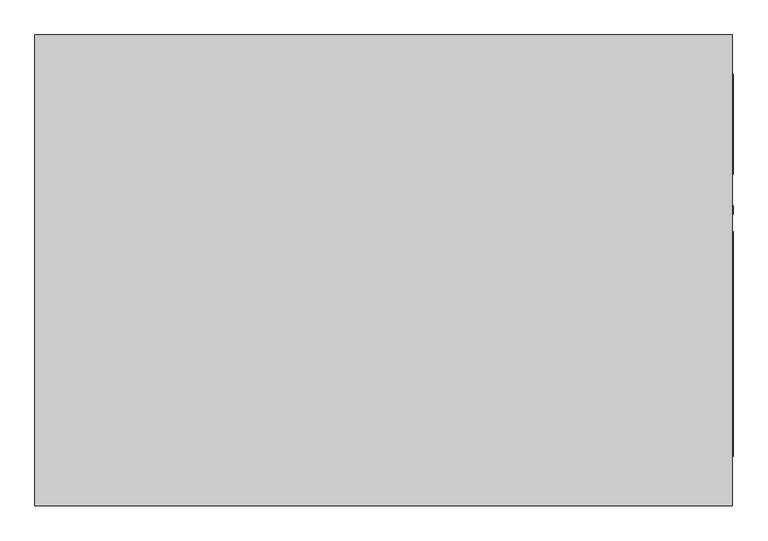
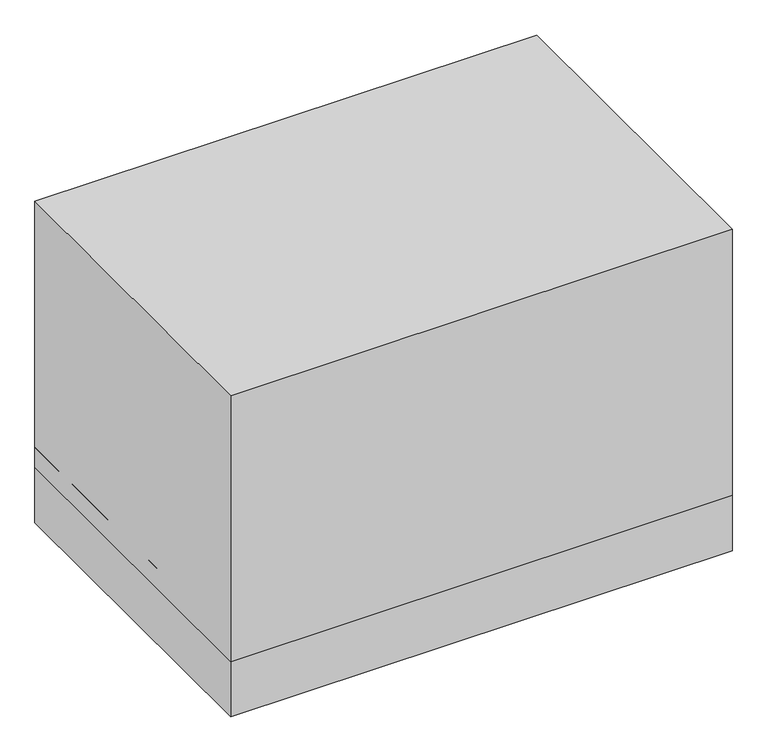
"""IFC4 building model written with IfcOpenShell, lengths in millimetres: proxy geometry, Carrier_48TC_Standard_Efficiency_Gas_Heat_Electric_Cooling_Packaged_Rooftop_Unit_3_to_15_nominal_tons : 10 ton 48TC**12."""

from ifc_helpers import new_model, si_unit, point, frame, frame_2d, origin, origin_with_axes, place, context, project, spatial, polyline, circle_curve, trimmed, segment, composite_curve, outline, extrude, source, transform, mapped, element, save
from ifc_brep_helpers import plane_surface, revolved_surface, advanced_brep


def mechanical_equipment_e741c091(model_context):
    return source(origin(), model_context, "Body", "SolidModel", [
        extrude(outline(composite_curve([segment(trimmed(circle_curve(frame_2d((193.675, 438.15)), 13.2953125), [point((180.3796875, 438.15))], [point((206.9703125, 438.15))], False, "CARTESIAN"), True, "CONTINUOUS"), segment(trimmed(circle_curve(frame_2d((193.675, 438.15)), 13.2953125), [point((206.9703125, 438.15))], [point((180.3796875, 438.15))], False, "CARTESIAN"), True, "CONTINUOUS")], self_intersect=False)), frame((1119.1875, 0.0, 0.0), z_axis=(1.0, 0.0, 0.0), x_axis=(0.0, 1.0, 0.0)), (0.0, 0.0, 1.0), 3.175),
        advanced_brep(
        [(1119.1875, 755.65, 1514.475), (-1119.1875, 755.65, 1514.475), (-1119.1875, -755.65, 1514.475), (1119.1875, -755.65, 1514.475), (1119.1875, 755.65, 260.35), (1119.1875, -755.65, 260.35), (-1119.1875, -755.65, 260.35), (-1119.1875, 755.65, 260.35), (1036.6375, -596.9, 260.35), (1036.6375, 133.35, 260.35), (681.0375, 133.35, 260.35), (681.0375, -596.9, 260.35), (1036.6375, 590.55, 260.35), (112.7125, 590.55, 260.35), (112.7125, 269.875, 260.35), (1036.6375, 269.875, 260.35), (176.8078125, -107.95, 260.35), (150.2171875, -107.95, 260.35), (-355.6, -476.25, 260.35), (-377.825, -476.25, 260.35), (-344.4875, -349.25, 260.35), (-388.9375, -349.25, 260.35), (-344.4875, -298.45, 260.35), (-388.9375, -298.45, 260.35), (1036.6375, -596.9, 381.0), (681.0375, -596.9, 381.0), (681.0375, 133.35, 381.0), (1036.6375, 133.35, 381.0), (1036.6375, 590.55, 381.0), (1036.6375, 269.875, 381.0), (112.7125, 269.875, 381.0), (112.7125, 590.55, 381.0), (176.8078125, -107.95, 406.4), (150.2171875, -107.95, 406.4), (-355.6, -476.25, 406.4), (-377.825, -476.25, 406.4), (-344.4875, -349.25, 406.4), (-388.9375, -349.25, 406.4), (-344.4875, -298.45, 406.4), (-388.9375, -298.45, 406.4)],
        [
            (0, 1),
            (1, 2),
            (2, 3),
            (3, 0),
            (4, 5),
            (5, 6),
            (6, 7),
            (7, 4),
            (8, 9),
            (9, 10),
            (10, 11),
            (11, 8),
            (12, 13),
            (13, 14),
            (14, 15),
            (15, 12),
            (16, 17, circle_curve(frame((163.5125, -107.95, 260.35), z_axis=(0.0, 0.0, 1.0), x_axis=(-1.0, 0.0, 0.0)), 13.2953125)),
            (17, 16, circle_curve(frame((163.5125, -107.95, 260.35), z_axis=(0.0, 0.0, 1.0), x_axis=(-1.0, 0.0, 0.0)), 13.2953125)),
            (18, 19, circle_curve(frame((-366.7125, -476.25, 260.35), z_axis=(0.0, 0.0, 1.0), x_axis=(-1.0, 0.0, 0.0)), 11.1125)),
            (19, 18, circle_curve(frame((-366.7125, -476.25, 260.35), z_axis=(0.0, 0.0, 1.0), x_axis=(-1.0, 0.0, 0.0)), 11.1125)),
            (20, 21, circle_curve(frame((-366.7125, -349.25, 260.35), z_axis=(0.0, 0.0, 1.0), x_axis=(-1.0, 0.0, 0.0)), 22.225)),
            (21, 20, circle_curve(frame((-366.7125, -349.25, 260.35), z_axis=(0.0, 0.0, 1.0), x_axis=(-1.0, 0.0, 0.0)), 22.225)),
            (22, 23, circle_curve(frame((-366.7125, -298.45, 260.35), z_axis=(0.0, 0.0, 1.0), x_axis=(-1.0, 0.0, 0.0)), 22.225)),
            (23, 22, circle_curve(frame((-366.7125, -298.45, 260.35), z_axis=(0.0, 0.0, 1.0), x_axis=(-1.0, 0.0, 0.0)), 22.225)),
            (0, 4),
            (7, 1),
            (6, 2),
            (5, 3),
            (24, 25),
            (25, 26),
            (26, 27),
            (27, 24),
            (27, 9),
            (8, 24),
            (26, 10),
            (25, 11),
            (28, 29),
            (29, 30),
            (30, 31),
            (31, 28),
            (31, 13),
            (12, 28),
            (30, 14),
            (29, 15),
            (32, 33, circle_curve(frame((163.5125, -107.95, 406.4), z_axis=(0.0, 0.0, -1.0), x_axis=(-1.0, 0.0, 0.0)), 13.2953125)),
            (33, 32, circle_curve(frame((163.5125, -107.95, 406.4), z_axis=(0.0, 0.0, -1.0), x_axis=(-1.0, 0.0, 0.0)), 13.2953125)),
            (33, 17),
            (16, 32),
            (34, 35, circle_curve(frame((-366.7125, -476.25, 406.4), z_axis=(0.0, 0.0, -1.0), x_axis=(-1.0, 0.0, 0.0)), 11.1125)),
            (35, 34, circle_curve(frame((-366.7125, -476.25, 406.4), z_axis=(0.0, 0.0, -1.0), x_axis=(-1.0, 0.0, 0.0)), 11.1125)),
            (35, 19),
            (18, 34),
            (36, 37, circle_curve(frame((-366.7125, -349.25, 406.4), z_axis=(0.0, 0.0, -1.0), x_axis=(-1.0, 0.0, 0.0)), 22.225)),
            (37, 36, circle_curve(frame((-366.7125, -349.25, 406.4), z_axis=(0.0, 0.0, -1.0), x_axis=(-1.0, 0.0, 0.0)), 22.225)),
            (37, 21),
            (20, 36),
            (38, 39, circle_curve(frame((-366.7125, -298.45, 406.4), z_axis=(0.0, 0.0, -1.0), x_axis=(-1.0, 0.0, 0.0)), 22.225)),
            (39, 38, circle_curve(frame((-366.7125, -298.45, 406.4), z_axis=(0.0, 0.0, -1.0), x_axis=(-1.0, 0.0, 0.0)), 22.225)),
            (39, 23),
            (22, 38),
        ],
        [
            plane_surface(frame((-1119.1875, 755.65, 1514.475), z_axis=(0.0, 0.0, 1.0), x_axis=(-1.0, 0.0, 0.0))),
            plane_surface(frame((-1119.1875, 755.65, 260.35), z_axis=(0.0, 0.0, -1.0), x_axis=(1.0, 0.0, 0.0))),
            plane_surface(frame((1119.1875, 755.65, 1514.475), z_axis=(0.0, 1.0, 0.0), x_axis=(0.0, 0.0, -1.0))),
            plane_surface(frame((-1119.1875, 755.65, 1514.475), z_axis=(-1.0, 0.0, 0.0), x_axis=(0.0, 0.0, -1.0))),
            plane_surface(frame((-1119.1875, -755.65, 1514.475), z_axis=(0.0, -1.0, 0.0), x_axis=(0.0, 0.0, -1.0))),
            plane_surface(frame((1119.1875, -755.65, 1514.475), z_axis=(1.0, 0.0, 0.0), x_axis=(0.0, 0.0, -1.0))),
            plane_surface(frame((1036.6375, -596.9, 381.0), z_axis=(0.0, 0.0, -1.0), x_axis=(0.0, 1.0, 0.0))),
            plane_surface(frame((1036.6375, -596.9, 381.0), z_axis=(-1.0, 0.0, 0.0), x_axis=(0.0, 0.0, -1.0))),
            plane_surface(frame((1036.6375, 133.35, 381.0), z_axis=(0.0, -1.0, 0.0), x_axis=(0.0, 0.0, -1.0))),
            plane_surface(frame((681.0375, 133.35, 381.0), z_axis=(1.0, 0.0, 0.0), x_axis=(0.0, 0.0, -1.0))),
            plane_surface(frame((681.0375, -596.9, 381.0), z_axis=(0.0, 1.0, 0.0), x_axis=(0.0, 0.0, -1.0))),
            plane_surface(frame((112.7125, 590.55, 381.0), z_axis=(0.0, 0.0, -1.0), x_axis=(-1.0, 0.0, 0.0))),
            plane_surface(frame((1036.6375, 590.55, 381.0), z_axis=(0.0, -1.0, 0.0), x_axis=(0.0, 0.0, -1.0))),
            plane_surface(frame((112.7125, 590.55, 381.0), z_axis=(1.0, 0.0, 0.0), x_axis=(0.0, 0.0, -1.0))),
            plane_surface(frame((112.7125, 269.875, 381.0), z_axis=(0.0, 1.0, 0.0), x_axis=(0.0, 0.0, -1.0))),
            plane_surface(frame((1036.6375, 269.875, 381.0), z_axis=(-1.0, 0.0, 0.0), x_axis=(0.0, 0.0, -1.0))),
            plane_surface(frame((150.2171875, -107.95, 406.4), z_axis=(0.0, 0.0, -1.0), x_axis=(0.0, -1.0, 0.0))),
            revolved_surface(polyline([(150.2171875, -107.95, 406.4), (150.2171875, -107.95, 260.35)]), (163.5125, -107.95, 0.0), (0.0, 0.0, 1.0)),
            plane_surface(frame((-377.825, -476.25, 406.4), z_axis=(0.0, 0.0, -1.0), x_axis=(0.0, -1.0, 0.0))),
            revolved_surface(polyline([(-377.825, -476.25, 406.4), (-377.825, -476.25, 260.35)]), (-366.7125, -476.25, 0.0), (0.0, 0.0, 1.0)),
            plane_surface(frame((-388.9375, -349.25, 406.4), z_axis=(0.0, 0.0, -1.0), x_axis=(0.0, -1.0, 0.0))),
            revolved_surface(polyline([(-388.9375, -349.25, 406.4), (-388.9375, -349.25, 260.35)]), (-366.7125, -349.25, 0.0), (0.0, 0.0, 1.0)),
            plane_surface(frame((-388.9375, -298.45, 406.4), z_axis=(0.0, 0.0, -1.0), x_axis=(0.0, -1.0, 0.0))),
            revolved_surface(polyline([(-388.9375, -298.45, 406.4), (-388.9375, -298.45, 260.35)]), (-366.7125, -298.45, 0.0), (0.0, 0.0, 1.0)),
        ],
        [
            (0, [[1, 2, 3, 4]]),
            (1, [[5, 6, 7, 8], [9, 10, 11, 12], [13, 14, 15, 16], [17, 18], [19, 20], [21, 22], [23, 24]]),
            (2, [[-1, 25, -8, 26]]),
            (3, [[-2, -26, -7, 27]]),
            (4, [[-3, -27, -6, 28]]),
            (5, [[-4, -28, -5, -25]]),
            (6, [[29, 30, 31, 32]]),
            (7, [[-32, 33, -9, 34]]),
            (8, [[-31, 35, -10, -33]]),
            (9, [[-30, 36, -11, -35]]),
            (10, [[-29, -34, -12, -36]]),
            (11, [[37, 38, 39, 40]]),
            (12, [[-40, 41, -13, 42]]),
            (13, [[-39, 43, -14, -41]]),
            (14, [[-38, 44, -15, -43]]),
            (15, [[-37, -42, -16, -44]]),
            (16, [[45, 46]]),
            (17, [[-46, 47, -17, 48]]),
            (17, [[-45, -48, -18, -47]]),
            (18, [[49, 50]]),
            (19, [[-50, 51, -19, 52]]),
            (19, [[-49, -52, -20, -51]]),
            (20, [[53, 54]]),
            (21, [[-54, 55, -21, 56]]),
            (21, [[-53, -56, -22, -55]]),
            (22, [[57, 58]]),
            (23, [[-58, 59, -23, 60]]),
            (23, [[-57, -60, -24, -59]]),
        ],
    ),
        extrude(outline(polyline([(1119.1875, 755.65), (1119.1875, -755.65), (-1119.1875, -755.65), (-1119.1875, 755.65), (1119.1875, 755.65)]), holes=[polyline([(1036.6375, 590.55), (112.7125, 590.55), (112.7125, 269.875), (1036.6375, 269.875), (1036.6375, 590.55)]), polyline([(1036.6375, -596.9), (1036.6375, 133.35), (681.0375, 133.35), (681.0375, -596.9), (1036.6375, -596.9)]), composite_curve([segment(trimmed(circle_curve(frame_2d((163.5125, -107.95)), 13.2953125), [point((176.8078125, -107.95))], [point((150.2171875, -107.95))], True, "CARTESIAN"), True, "CONTINUOUS"), segment(trimmed(circle_curve(frame_2d((163.5125, -107.95)), 13.2953125), [point((150.2171875, -107.95))], [point((176.8078125, -107.95))], True, "CARTESIAN"), True, "CONTINUOUS")], self_intersect=False), composite_curve([segment(trimmed(circle_curve(frame_2d((-366.7125, -476.25)), 11.1125), [point((-355.6, -476.25))], [point((-377.825, -476.25))], True, "CARTESIAN"), True, "CONTINUOUS"), segment(trimmed(circle_curve(frame_2d((-366.7125, -476.25)), 11.1125), [point((-377.825, -476.25))], [point((-355.6, -476.25))], True, "CARTESIAN"), True, "CONTINUOUS")], self_intersect=False), composite_curve([segment(trimmed(circle_curve(frame_2d((-366.7125, -349.25)), 22.225), [point((-344.4875, -349.25))], [point((-388.9375, -349.25))], True, "CARTESIAN"), True, "CONTINUOUS"), segment(trimmed(circle_curve(frame_2d((-366.7125, -349.25)), 22.225), [point((-388.9375, -349.25))], [point((-344.4875, -349.25))], True, "CARTESIAN"), True, "CONTINUOUS")], self_intersect=False), composite_curve([segment(trimmed(circle_curve(frame_2d((-366.7125, -298.45)), 22.225), [point((-344.4875, -298.45))], [point((-388.9375, -298.45))], True, "CARTESIAN"), True, "CONTINUOUS"), segment(trimmed(circle_curve(frame_2d((-366.7125, -298.45)), 22.225), [point((-388.9375, -298.45))], [point((-344.4875, -298.45))], True, "CARTESIAN"), True, "CONTINUOUS")], self_intersect=False)]), origin_with_axes(), (0.0, 0.0, 1.0), 355.6),
        extrude(outline(polyline([(1122.3625, 628.65), (1122.3625, 307.975), (1119.1875, 307.975), (1119.1875, 628.65), (1122.3625, 628.65)])), frame((0.0, 0.0, 406.4), z_axis=(0.0, 0.0, 1.0), x_axis=(1.0, 0.0, 0.0)), (0.0, 0.0, 1.0), 923.925),
        extrude(outline(polyline([(1122.3625, 123.825), (1122.3625, -596.9), (1119.1875, -596.9), (1119.1875, 123.825), (1122.3625, 123.825)])), frame((0.0, 0.0, 406.4), z_axis=(0.0, 0.0, 1.0), x_axis=(1.0, 0.0, 0.0)), (0.0, 0.0, 1.0), 352.425),
    ])


if __name__ == "__main__":
    model = new_model("IFC4")
    model_context = context("Model", 3, world=origin())
    ifc_project = project(units=[si_unit("LENGTHUNIT", "METRE", prefix="MILLI")], contexts=[model_context])
    site = spatial("IfcSite", under=ifc_project)
    building = spatial("IfcBuilding", under=site)
    placement = place(None, origin())
    mechanical_equipment_shape = mechanical_equipment_e741c091(model_context)
    element("IfcBuildingElementProxy", 1, Name="Carrier_48TC_Standard_Efficiency_Gas_Heat_Electric_Cooling_Packaged_Rooftop_Unit_3_to_15_nominal_tons : 10 ton 48TC**12", ObjectType="Carrier_48TC_Standard_Efficiency_Gas_Heat_Electric_Cooling_Packaged_Rooftop_Unit_3_to_15_nominal_tons : 10 ton 48TC**12", at=placement, inside=building, context=model_context, shape_type="MappedRepresentation", body=[
        mapped(mechanical_equipment_shape, transform((0.0, 0.0, 0.0), x_axis=(1.0, 0.0, 0.0), y_axis=(0.0, 1.0, 0.0), z_axis=(0.0, 0.0, 1.0))),
    ])
    save(model, "model.ifc")

# Revit data of these elements
# Type "Carrier_48TC_Standard_Efficiency_Gas_Heat_Electric_Cooling_Packaged_Rooftop_Unit_3_to_15_nominal_tons : 10 ton 48TC**12"
#   URL = "www.Carrier.com"
#   Model = "48TC"
#   Manufacturer = "Carrier"
#   Disclaimer = "Manufacturer reserves the right to change, at any time, specifications and designs without notice and without obligation.  Please verify critical parameters with local Carrier commercial sales office."
#   knockout thickness = 0' - 0 1/16"
#   Voltage = 0 V
#   Version = 1
#   TTBY3 = 0' - 11"
#   TTBY2 = 1' - 4"
#   TTBY1 = 1' - 6"
#   TTBX = 2' - 5 5/8"
#   TTBPowerR = 0' - 0 7/8"
#   TTBGasR = 0' - 0 7/8"
#   SSSZ = 0' - 5 3/4"
#   SSSY = 0' - 6 1/4"
#   SSSW = 2' - 4 3/8"
#   SSSH = 1' - 1 7/8"
#   SSRZ = 0' - 5 3/4"
#   SSRY = 0' - 5"
#   SSRW = 1' - 0 5/8"
#   SSRH = 3' - 0 3/8"
#   SEER = 0
#   Right clearance = 3' - 0"
#   PWRZ = 2' - 3 7/8"
#   PWRY = 0' - 4 5/8"
#   PWRR = 0' - 1 1/4"
#   ODF2X = 1' - 0"
#   ODF1Y = 0' - 11"
#   ODF1X = 2' - 1"
#   ODF1R = 0' - 10"
#   MOCP = 0 A
#   MCA = 0 A
#   Left clearance = 4' - 0"
#   IEER = 11.8
#   Front clearance = 4' - 0"
#   Fan Z = 4' - 11 5/8"
#   Width = 4' - 11 1/2"
#   Length = 7' - 4 1/8"
#   Height = 4' - 1 3/8"
#   EER = 11.1
#   DSSY = 0' - 6 1/4"
#   DSSX = 0' - 3 1/4"
#   DSSW = 1' - 2"
#   DSSH = 2' - 4 3/4"
#   DSRY = 0' - 6 1/2"
#   DSRX = 0' - 3 1/4"
#   DSRW = 3' - 0 3/8"
#   DSRH = 1' - 0 5/8"
#   DRNZ = 0' - 7"
#   DRNY = 3' - 1 3/8"
#   DRNR = 0' - 0 67/128"
#   Curb Z = 1' - 2"
#   CFM (nominal) = 0 CFM
#   Back clearance = 3' - 0"
#   Alt Condensate Drain = 0' - 0 67/128"
#   AccypwrR = 0' - 0 7/16"
#   ACY = 2' - 1 1/2"
#   ACX = 3' - 1 5/8"
#   Gas [instance default] = yes
#   Fan 2 on = yes
#   Curb_1SLAB_2ROOFCURB_3SNOWCURB = 2
#   Fan 3 on = no
#   Unit material = RTU
#   Curb material = Curb paint
# Element 1 (IfcBuildingElementProxy, "Carrier_48TC_Standard_Efficiency_Gas_Heat_Electric_Cooling_Packaged_Rooftop_Unit_3_to_15_nominal_tons : 10 ton 48TC**12")
#   Materials on its faces: "RTU", "Curb paint", "Mech"
# Materials
#   "RTU": class "Miscellaneous", colour RGB 104 104 104, transparency 0, Cost = 0
#   "Curb paint": class "Miscellaneous", colour RGB 189 187 185, transparency 0
#   "Mech": class "Miscellaneous", colour RGB 235 237 235, transparency 0, Cost = 0
